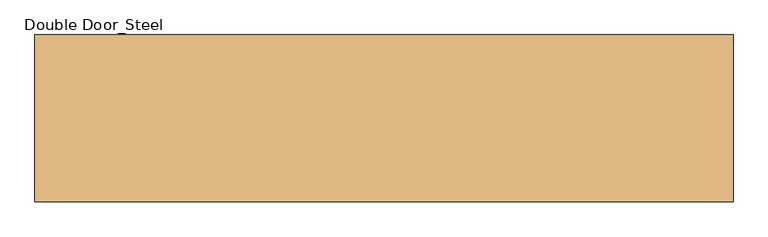
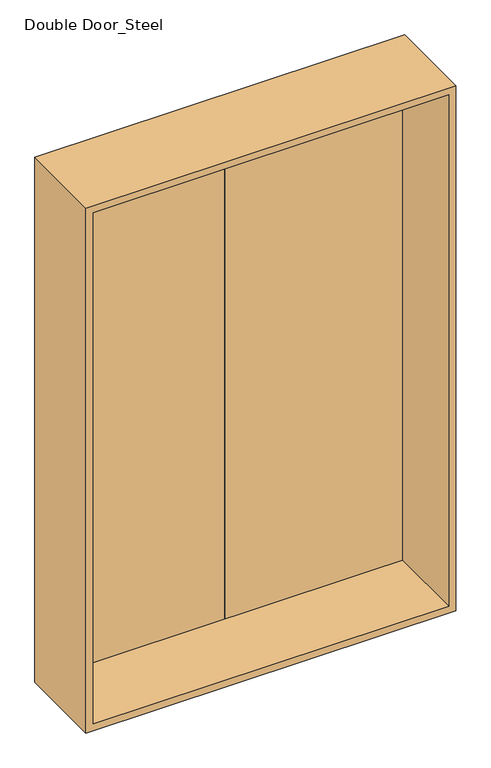
"""IFC4 building model written with IfcOpenShell, lengths in millimetres: door geometry, Double Door_Steel : H_DR_AMB_Double Door_Steel_W1800xH2700."""

import ifcopenshell
import ifcopenshell.guid

model = None  # the IFC model being written
_history = None  # IfcOwnerHistory: only IFC2X3 demands one
_inside = {}  # id of a spatial element -> (the spatial element, [elements in it])
_under = {}  # id of a project, library or spatial element -> (it, [spatial elements below it])
_declared = {}  # id of a project -> (the project, [libraries it declares])
_typed = {}  # id of a type object -> (the type object, [elements of that type])
_made_of = {}  # id of a material, layer set ... -> (it, [elements and type objects made of it])


def new_model(schema):
    """Start an empty IFC model of exactly this schema.

    Asked for "IFC4X3", IfcOpenShell would pick the latest addendum, in which some entities
    have other attributes; the version numbers below select the first issue.
    IFC2X3 requires an IfcOwnerHistory on every rooted entity: one is made here for all.
    """
    global model, _history
    if schema == "IFC4X3":
        model = ifcopenshell.file(schema_version=(4, 3, 0, 0))
    else:
        model = ifcopenshell.file(schema=schema)
    _inside.clear()
    _under.clear()
    _declared.clear()
    _typed.clear()
    _made_of.clear()
    _history = None
    if model.schema == "IFC2X3":
        org = make("IfcOrganization", Name="unknown")
        user = make(
            "IfcPersonAndOrganization",
            ThePerson=make("IfcPerson", FamilyName="unknown"),
            TheOrganization=org,
        )
        app = make(
            "IfcApplication",
            ApplicationDeveloper=org,
            Version="unknown",
            ApplicationFullName="unknown",
            ApplicationIdentifier="unknown",
        )
        _history = make(
            "IfcOwnerHistory",
            OwningUser=user,
            OwningApplication=app,
            ChangeAction="ADDED",
            CreationDate=0,
        )
    return model


def make(cls, **values):
    """One entity of the class cls with the attributes given. An attribute that is None is left unset."""
    return model.create_entity(
        cls, **{name: value for name, value in values.items() if value is not None}
    )


def rooted(cls, **values):
    """An entity with a GlobalId (a new one), such as an element, a storey or a relation."""
    return make(cls, GlobalId=ifcopenshell.guid.new(), OwnerHistory=_history, **values)


def si_unit(unit_type, name, prefix=None):
    """IfcSIUnit, for example si_unit("LENGTHUNIT", "METRE", prefix="MILLI")."""
    return make("IfcSIUnit", UnitType=unit_type, Prefix=prefix, Name=name)


def assignment(units):
    """IfcUnitAssignment: the units of a project."""
    return None if units is None else make("IfcUnitAssignment", Units=units)


def point(xyz):
    """IfcCartesianPoint."""
    return None if xyz is None else make("IfcCartesianPoint", Coordinates=xyz)


def direction(xyz):
    """IfcDirection."""
    return None if xyz is None else make("IfcDirection", DirectionRatios=xyz)


def frame(location, z_axis=None, x_axis=None):
    """IfcAxis2Placement3D, a coordinate frame: its origin and axes. An axis left out is left unset."""
    return make(
        "IfcAxis2Placement3D",
        Location=point(location),
        Axis=direction(z_axis),
        RefDirection=direction(x_axis),
    )


def origin():
    """The frame at (0, 0, 0) with its axes left unset."""
    return frame((0.0, 0.0, 0.0))


def place(relative_to, where):
    """IfcLocalPlacement: puts the frame where relative to a parent placement (None: the world)."""
    return make(
        "IfcLocalPlacement", PlacementRelTo=relative_to, RelativePlacement=where
    )


def context(
    kind, dimensions, precision=None, world=None, true_north=None, identifier=None
):
    """IfcGeometricRepresentationContext, for example the 3D "Model" context."""
    return make(
        "IfcGeometricRepresentationContext",
        ContextIdentifier=identifier,
        ContextType=kind,
        CoordinateSpaceDimension=dimensions,
        Precision=precision,
        WorldCoordinateSystem=world,
        TrueNorth=true_north,
    )


def project(units=None, contexts=None):
    """IfcProject with its units and contexts."""
    return rooted(
        "IfcProject",
        Name="project",
        RepresentationContexts=contexts,
        UnitsInContext=assignment(units),
    )


def spatial(cls, under=None, at=None, **own):
    """A site, building, storey or space (cls), placed at a placement, below another one or the project."""
    s = rooted(cls, ObjectPlacement=at, **own)
    if under is not None:
        _under.setdefault(under.id(), (under, []))[1].append(s)
    return s


def polyline(points):
    """IfcPolyline through the points."""
    return make("IfcPolyline", Points=[point(p) for p in points])


def outline(outer, holes=None, kind="AREA"):
    """IfcArbitraryClosedProfileDef: a profile drawn as a closed curve; with holes, ...WithVoids."""
    if holes is None:
        return make("IfcArbitraryClosedProfileDef", ProfileType=kind, OuterCurve=outer)
    return make(
        "IfcArbitraryProfileDefWithVoids",
        ProfileType=kind,
        OuterCurve=outer,
        InnerCurves=holes,
    )


def extrude(swept, where, along, depth):
    """IfcExtrudedAreaSolid: the profile swept, set in the frame where, extruded along a direction by depth."""
    return make(
        "IfcExtrudedAreaSolid",
        SweptArea=swept,
        Position=where,
        ExtrudedDirection=direction(along),
        Depth=depth,
    )


def faces_of(points, faces, orient=None, outer=None):
    """IfcFace entities. A face is a list of loops; a loop is a list of indices into points, from 0.

    orient and outer hold one flag for each loop. By default every Orientation is true, the
    first loop of a face is its IfcFaceOuterBound and the others are IfcFaceBound.
    """
    made = []
    for i, loops in enumerate(faces):
        bounds = []
        for j, loop in enumerate(loops):
            is_outer = j == 0 if outer is None else outer[i][j]
            bounds.append(
                make(
                    "IfcFaceOuterBound" if is_outer else "IfcFaceBound",
                    Bound=make("IfcPolyLoop", Polygon=[points[k] for k in loop]),
                    Orientation=True if orient is None else orient[i][j],
                )
            )
        made.append(make("IfcFace", Bounds=bounds))
    return made


def faceted_brep(points, faces, orient=None, outer=None, voids=None):
    """IfcFacetedBrep: a solid bounded by flat faces; with voids (closed shells), ...WithVoids."""
    shared = [point(p) for p in points]
    hull = make("IfcClosedShell", CfsFaces=faces_of(shared, faces, orient, outer))
    if voids is None:
        return make("IfcFacetedBrep", Outer=hull)
    return make(
        "IfcFacetedBrepWithVoids",
        Outer=hull,
        Voids=[
            make(cls, CfsFaces=faces_of(shared, fs, o, b)) for cls, fs, o, b in voids
        ],
    )


def shape(context_of_items, identifier, shape_type, items):
    """IfcShapeRepresentation: the items that make up one representation, for example the "Body"."""
    return make(
        "IfcShapeRepresentation",
        ContextOfItems=context_of_items,
        RepresentationIdentifier=identifier,
        RepresentationType=shape_type,
        Items=items,
    )


def source(mapping_origin, context_of_items, identifier, shape_type, items):
    """IfcRepresentationMap: a shape defined once, which mapped items show again and again."""
    return make(
        "IfcRepresentationMap",
        MappingOrigin=mapping_origin,
        MappedRepresentation=shape(context_of_items, identifier, shape_type, items),
    )


def transform(
    local_origin,
    x_axis=None,
    y_axis=None,
    z_axis=None,
    scale=None,
    scale2=None,
    scale3=None,
    uniform=True,
):
    """IfcCartesianTransformationOperator3D, or its non-uniform kind. x_axis, y_axis, z_axis: its Axis1, 2, 3."""
    if uniform:
        return make(
            "IfcCartesianTransformationOperator3D",
            Axis1=direction(x_axis),
            Axis2=direction(y_axis),
            LocalOrigin=point(local_origin),
            Scale=scale,
            Axis3=direction(z_axis),
        )
    return make(
        "IfcCartesianTransformationOperator3DnonUniform",
        Axis1=direction(x_axis),
        Axis2=direction(y_axis),
        LocalOrigin=point(local_origin),
        Scale=scale,
        Axis3=direction(z_axis),
        Scale2=scale2,
        Scale3=scale3,
    )


def mapped(mapping_source, mapping_target):
    """IfcMappedItem: shows the shape of a source again, moved by a transform."""
    return make(
        "IfcMappedItem", MappingSource=mapping_source, MappingTarget=mapping_target
    )


def made_of(thing, what):
    """Note that an element or type object is made of a material, layer set ...; save() writes the relation."""
    if what is not None:
        _made_of.setdefault(what.id(), (what, []))[1].append(thing)
    return thing


def element(
    cls,
    number,
    at=None,
    inside=None,
    cuts=None,
    type_object=None,
    material=None,
    context=None,
    identifier="Body",
    shape_type=None,
    held_by="IfcProductDefinitionShape",
    body=None,
    shapes=None,
    **own,
):
    """One element of the class cls, such as IfcWall. Its Tag is "e" and its number.

    at: its placement. inside: the storey or other place that contains it. cuts: it is an
    opening in that element (IfcRelVoidsElement). A single representation is given by context,
    identifier, shape_type and body (its items); several are given by shapes. held_by: the class
    of the entity that holds the representations. save() writes the other relations.
    """
    e = rooted(cls, Tag="e%d" % number, ObjectPlacement=at, **own)
    if body is not None:
        shapes = [shape(context, identifier, shape_type, body)]
    if shapes is not None:
        e.Representation = make(held_by, Representations=shapes)
    if inside is not None:
        _inside.setdefault(inside.id(), (inside, []))[1].append(e)
    if cuts is not None:
        rooted(
            "IfcRelVoidsElement", RelatingBuildingElement=cuts, RelatedOpeningElement=e
        )
    if type_object is not None:
        _typed.setdefault(type_object.id(), (type_object, []))[1].append(e)
    return made_of(e, material)


def aggregate(whole, parts):
    """IfcRelAggregates: a whole, such as a stair, and the parts it consists of."""
    return rooted("IfcRelAggregates", RelatingObject=whole, RelatedObjects=parts)


def save(model, path):
    """Write the relations noted so far, then the file.

    IfcRelAggregates (storeys below a building ...), IfcRelContainedInSpatialStructure (elements
    in a storey), IfcRelDefinesByType, IfcRelAssociatesMaterial and IfcRelDeclares: one each for
    every whole, place, type object, material and project.
    """
    for whole, parts in _under.values():
        aggregate(whole, parts)
    for where, things in _inside.values():
        rooted(
            "IfcRelContainedInSpatialStructure",
            RelatedElements=things,
            RelatingStructure=where,
        )
    for kind, things in _typed.values():
        rooted("IfcRelDefinesByType", RelatedObjects=things, RelatingType=kind)
    for what, things in _made_of.values():
        rooted("IfcRelAssociatesMaterial", RelatedObjects=things, RelatingMaterial=what)
    for by, libraries in _declared.values():
        rooted("IfcRelDeclares", RelatingContext=by, RelatedDefinitions=libraries)
    model.write(path)


def double_door_steel_634f6038(model_context):
    return source(origin(), model_context, "Body", "SolidModel", [
        extrude(outline(polyline([(880.0, 175.0), (0.0, 175.0), (0.0, 215.0), (880.0, 215.0), (880.0, 175.0)])), frame((0.0, 0.0, 20.0), z_axis=(0.0, 0.0, 1.0), x_axis=(1.0, 0.0, 0.0)), (0.0, 0.0, 1.0), 2660.0),
        extrude(outline(polyline([(0.0, 175.0), (-880.0, 175.0), (-880.0, 215.0), (0.0, 215.0), (0.0, 175.0)])), frame((0.0, 0.0, 20.0), z_axis=(0.0, 0.0, 1.0), x_axis=(1.0, 0.0, 0.0)), (0.0, 0.0, 1.0), 2660.0),
        faceted_brep([(900.0, -215.0, 2700.0), (900.0, 215.0, 2700.0), (-900.0, 215.0, 2700.0), (-900.0, -215.0, 2700.0), (865.0, 175.0, 2665.0), (865.0, -215.0, 2665.0), (-865.0, -215.0, 2665.0), (-865.0, 175.0, 2665.0), (880.0, 215.0, 2680.0), (880.0, 175.0, 2680.0), (-880.0, 175.0, 2680.0), (-880.0, 215.0, 2680.0), (-900.0, 215.0, 0.0), (-900.0, -215.0, 0.0), (-865.0, -215.0, 35.0), (-865.0, 175.0, 35.0), (-880.0, 175.0, 20.0), (-880.0, 215.0, 20.0), (900.0, 215.0, 0.0), (880.0, 215.0, 20.0), (900.0, -215.0, 0.0), (865.0, -215.0, 35.0), (865.0, 175.0, 35.0), (880.0, 175.0, 20.0)], [[[0, 1, 2, 3]], [[4, 5, 6, 7]], [[8, 9, 10, 11]], [[3, 2, 12, 13]], [[7, 6, 14, 15]], [[11, 10, 16, 17]], [[18, 12, 2, 1], [8, 11, 17, 19]], [[13, 12, 18, 20]], [[0, 3, 13, 20], [21, 14, 6, 5]], [[15, 14, 21, 22]], [[23, 16, 10, 9], [4, 7, 15, 22]], [[17, 16, 23, 19]], [[20, 18, 1, 0]], [[22, 21, 5, 4]], [[19, 23, 9, 8]]]),
    ])


if __name__ == "__main__":
    model = new_model("IFC4")
    model_context = context("Model", 3, world=origin())
    ifc_project = project(units=[si_unit("LENGTHUNIT", "METRE", prefix="MILLI")], contexts=[model_context])
    site = spatial("IfcSite", under=ifc_project)
    building = spatial("IfcBuilding", under=site)
    placement = place(None, origin())
    double_door_steel_shape = double_door_steel_634f6038(model_context)
    element("IfcDoor", 1, ObjectType="Double Door_Steel : H_DR_AMB_Double Door_Steel_W1800xH2700", at=placement, inside=building, context=model_context, shape_type="MappedRepresentation", body=[
        mapped(double_door_steel_shape, transform((0.0, 0.0, 0.0), x_axis=(1.0, 0.0, 0.0), y_axis=(0.0, 1.0, 0.0), z_axis=(0.0, 0.0, 1.0))),
    ])
    save(model, "model.ifc")

# Revit data of these elements
# Type "Double Door_Steel : H_DR_AMB_Double Door_Steel_W1800xH2700"
#   Type Mark = "363"
#   프레임 = ""
#   철물 = ""
#   유리/마감 = ""
#   위치/개소 = ""
#   부호 = "1/SD"
#   문번호 = ""
#   문기호 = "SD"
#   Analytic Construction = "<None>"
#   Height = 2700.000 mm
#   Width = 1800.000 mm
#   Define Thermal Properties by = 1
#   문 틀 = none
#   문 = none
#   Function = (empty or 0)
#   Assembly Code = ""
#   Wall Closure = (empty or 0)
